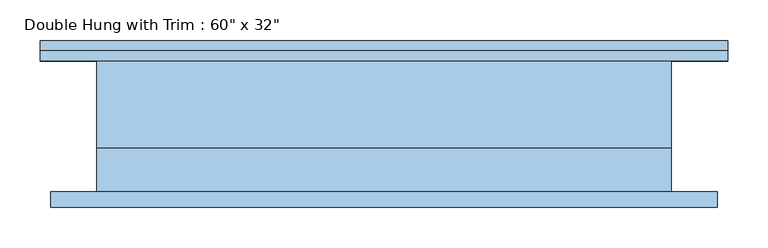
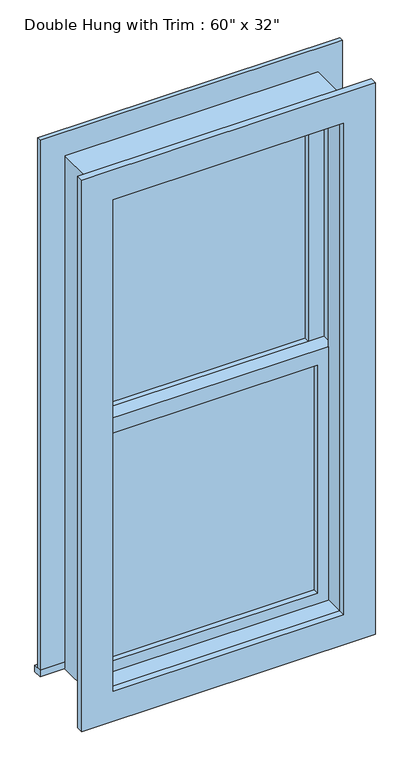
"""IFC4 building model written with IfcOpenShell, lengths in millimetres: window geometry."""

from ifc_helpers import new_model, si_unit, frame, origin, place, context, project, spatial, polyline, outline, extrude, source, transform, mapped, element, save


def window_c0f0d920(model_context):
    return source(origin(), model_context, "Body", "SweptSolid", [
        extrude(outline(polyline([(-292.1, 1.5875), (292.1, 1.5875), (292.1, -11.1125), (-292.1, -11.1125), (-292.1, 1.5875)])), frame((0.0, 0.0, 977.9), z_axis=(0.0, 0.0, 1.0), x_axis=(1.0, 0.0, 0.0)), (0.0, 0.0, 1.0), 676.275),
        extrude(outline(polyline([(1698.625, -336.55), (933.45, -336.55), (933.45, 336.55), (1698.625, 336.55), (1698.625, -336.55)]), holes=[polyline([(1654.175, -292.1), (1654.175, 292.1), (977.9, 292.1), (977.9, -292.1), (1654.175, -292.1)])]), frame((0.0, -26.9875, 0.0), z_axis=(0.0, 1.0, 0.0), x_axis=(0.0, 0.0, 1.0)), (0.0, 0.0, 1.0), 44.45),
        extrude(outline(polyline([(-425.45, 106.3625), (425.45, 106.3625), (425.45, 80.9625), (-425.45, 80.9625), (-425.45, 106.3625)])), frame((0.0, 0.0, 914.4), z_axis=(0.0, 0.0, 1.0), x_axis=(1.0, 0.0, 0.0)), (0.0, 0.0, 1.0), 19.05),
        extrude(outline(polyline([(2419.35, -336.55), (2419.35, 336.55), (933.45, 336.55), (933.45, 425.45), (2508.25, 425.45), (2508.25, -425.45), (933.45, -425.45), (933.45, -336.55), (2419.35, -336.55)])), frame((0.0, 80.9625, 0.0), z_axis=(0.0, 1.0, 0.0), x_axis=(0.0, 0.0, 1.0)), (0.0, 0.0, 1.0), 12.7),
        extrude(outline(polyline([(2495.55, 412.75), (2495.55, -412.75), (857.25, -412.75), (857.25, 412.75), (2495.55, 412.75)]), holes=[polyline([(2406.65, 323.85), (946.15, 323.85), (946.15, -323.85), (2406.65, -323.85), (2406.65, 323.85)])]), frame((0.0, -100.0125, 0.0), z_axis=(0.0, 1.0, 0.0), x_axis=(0.0, 0.0, 1.0)), (0.0, 0.0, 1.0), 19.05),
        extrude(outline(polyline([(292.1, 33.3375), (-292.1, 33.3375), (-292.1, 46.0375), (292.1, 46.0375), (292.1, 33.3375)])), frame((0.0, 0.0, 1698.625), z_axis=(0.0, 0.0, 1.0), x_axis=(1.0, 0.0, 0.0)), (0.0, 0.0, 1.0), 676.275),
        extrude(outline(polyline([(2419.35, -336.55), (1654.175, -336.55), (1654.175, 336.55), (2419.35, 336.55), (2419.35, -336.55)]), holes=[polyline([(2374.9, -292.1), (2374.9, 292.1), (1698.625, 292.1), (1698.625, -292.1), (2374.9, -292.1)])]), frame((0.0, 17.4625, 0.0), z_axis=(0.0, 1.0, 0.0), x_axis=(0.0, 0.0, 1.0)), (0.0, 0.0, 1.0), 44.45),
        extrude(outline(polyline([(2438.4, -355.6), (914.4, -355.6), (914.4, 355.6), (2438.4, 355.6), (2438.4, -355.6)]), holes=[polyline([(2406.65, -323.85), (2406.65, 323.85), (946.15, 323.85), (946.15, -323.85), (2406.65, -323.85)])]), frame((0.0, -80.9625, 0.0), z_axis=(0.0, 1.0, 0.0), x_axis=(0.0, 0.0, 1.0)), (0.0, 0.0, 1.0), 53.975),
        extrude(outline(polyline([(2438.4, 355.6), (2438.4, -355.6), (914.4, -355.6), (914.4, 355.6), (2438.4, 355.6)]), holes=[polyline([(2419.35, 336.55), (933.45, 336.55), (933.45, -336.55), (2419.35, -336.55), (2419.35, 336.55)])]), frame((0.0, -26.9875, 0.0), z_axis=(0.0, 1.0, 0.0), x_axis=(0.0, 0.0, 1.0)), (0.0, 0.0, 1.0), 107.95),
    ])


if __name__ == "__main__":
    model = new_model("IFC4")
    model_context = context("Model", 3, world=origin())
    ifc_project = project(units=[si_unit("LENGTHUNIT", "METRE", prefix="MILLI")], contexts=[model_context])
    site = spatial("IfcSite", under=ifc_project)
    building = spatial("IfcBuilding", under=site)
    placement = place(None, origin())
    window_shape = window_c0f0d920(model_context)
    element("IfcWindow", 1, ObjectType="Double Hung with Trim : 60\" x 32\"", at=placement, inside=building, context=model_context, shape_type="MappedRepresentation", body=[
        mapped(window_shape, transform((0.0, 0.0, 0.0), x_axis=(1.0, 0.0, 0.0), y_axis=(0.0, 1.0, 0.0), z_axis=(0.0, 0.0, 1.0))),
    ])
    save(model, "model.ifc")

# Revit data of these elements
# Type "Double Hung with Trim : 60\" x 32\""
#   Type Mark = "62"
#   COBie.Type.CreatedBy = "doug.wood@us.ibm.com"
#   COBie.Type.CreatedOn = "2016-04-14T02:07:26"
#   COBie.Type.Name = "Windows_Double Hung with Trim_60\" x 32\"_62"
#   COBie.Type.Category = "23-30 20 17 17 14 : Double-Hung Windows"
#   COBie.Type.Description = "Double Hung with Trim_60\" x 32\""
#   COBie.Type.Manufacturer = ""
#   COBie.Type.ModelNumber = ""
#   Construction Type Id = "GSP4R"
#   Assembly Code = "B2020100"
#   Analytic Construction = "1/8 in Pilkington single glazing"
#   COBie.Type.ReplacementCost = 0
#   Visual Light Transmittance = 0.9
#   Solar Heat Gain Coefficient = 0.78
#   Heat Transfer Coefficient (U) = 3.6886 W/(m²·K)
#   Height = 5' - 0"
#   Default Sill Height = 3' - 0"
#   Trim Projection - Ext. = 0' - 0 1/2"
#   Trim Projection - Int. = 0' - 0 3/4"
#   Trim Width - Exterior = 0' - 3 1/2"
#   Trim Width - Interior = 0' - 3 1/2"
#   Width = 2' - 4"
#   Window Inset = 0' - 0 3/4"
#   COBie.Type = no
#   Glass Pane Material = Glass
#   Sash Material = Sash - White
#   Trim Exterior Material = Trim - White
#   Trim Interior Material = Trim - White
#   Wall Closure = (empty or 0)
# Element 1 (IfcWindow, "Double Hung with Trim : 60\" x 32\"")
#   Materials on its faces: "Sash - White", "Trim - White", "Glass"
# Materials
#   "Glass": class "Glass", colour RGB 0 128 192, transparency 0.75, Description = "Soda Lime Glass", Cost = 0
#   "Sash - White": class "Wood", colour RGB 255 255 255, transparency 0, Cost = 0
#   "Trim - White": class "Wood", colour RGB 255 255 255, transparency 0, Cost = 0
